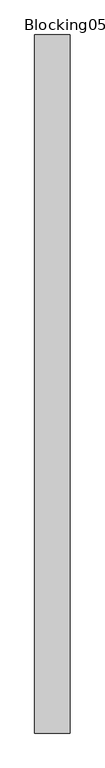
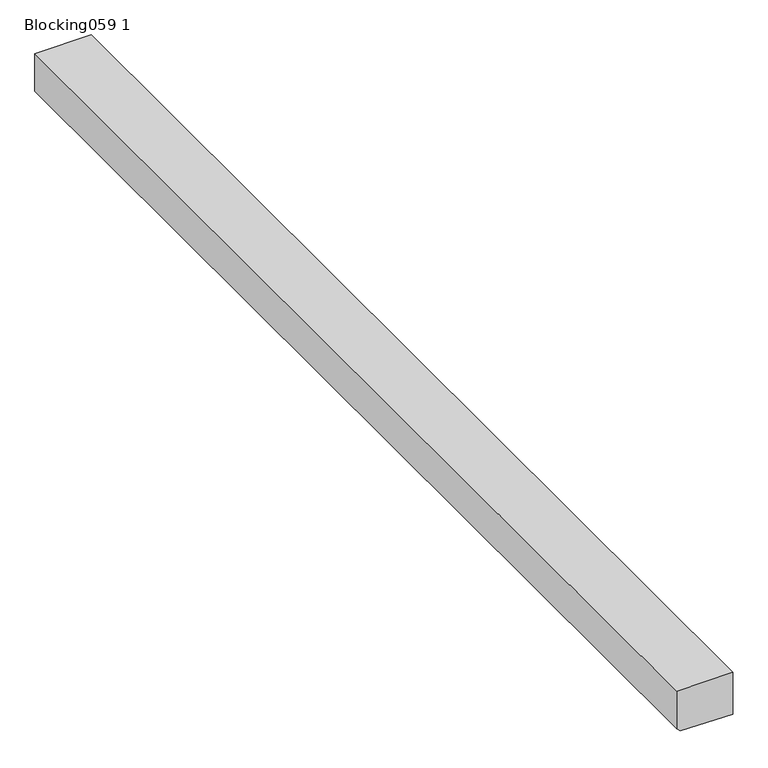
"""IFC4 building model written with IfcOpenShell, lengths in millimetres: proxy geometry, Blocking059 1 : Blocking059 1918."""

import ifcopenshell
import ifcopenshell.guid

model = None  # the IFC model being written
_history = None  # IfcOwnerHistory: only IFC2X3 demands one
_inside = {}  # id of a spatial element -> (the spatial element, [elements in it])
_under = {}  # id of a project, library or spatial element -> (it, [spatial elements below it])
_declared = {}  # id of a project -> (the project, [libraries it declares])
_typed = {}  # id of a type object -> (the type object, [elements of that type])
_made_of = {}  # id of a material, layer set ... -> (it, [elements and type objects made of it])


def new_model(schema):
    """Start an empty IFC model of exactly this schema.

    Asked for "IFC4X3", IfcOpenShell would pick the latest addendum, in which some entities
    have other attributes; the version numbers below select the first issue.
    IFC2X3 requires an IfcOwnerHistory on every rooted entity: one is made here for all.
    """
    global model, _history
    if schema == "IFC4X3":
        model = ifcopenshell.file(schema_version=(4, 3, 0, 0))
    else:
        model = ifcopenshell.file(schema=schema)
    _inside.clear()
    _under.clear()
    _declared.clear()
    _typed.clear()
    _made_of.clear()
    _history = None
    if model.schema == "IFC2X3":
        org = make("IfcOrganization", Name="unknown")
        user = make(
            "IfcPersonAndOrganization",
            ThePerson=make("IfcPerson", FamilyName="unknown"),
            TheOrganization=org,
        )
        app = make(
            "IfcApplication",
            ApplicationDeveloper=org,
            Version="unknown",
            ApplicationFullName="unknown",
            ApplicationIdentifier="unknown",
        )
        _history = make(
            "IfcOwnerHistory",
            OwningUser=user,
            OwningApplication=app,
            ChangeAction="ADDED",
            CreationDate=0,
        )
    return model


def make(cls, **values):
    """One entity of the class cls with the attributes given. An attribute that is None is left unset."""
    return model.create_entity(
        cls, **{name: value for name, value in values.items() if value is not None}
    )


def rooted(cls, **values):
    """An entity with a GlobalId (a new one), such as an element, a storey or a relation."""
    return make(cls, GlobalId=ifcopenshell.guid.new(), OwnerHistory=_history, **values)


def si_unit(unit_type, name, prefix=None):
    """IfcSIUnit, for example si_unit("LENGTHUNIT", "METRE", prefix="MILLI")."""
    return make("IfcSIUnit", UnitType=unit_type, Prefix=prefix, Name=name)


def assignment(units):
    """IfcUnitAssignment: the units of a project."""
    return None if units is None else make("IfcUnitAssignment", Units=units)


def point(xyz):
    """IfcCartesianPoint."""
    return None if xyz is None else make("IfcCartesianPoint", Coordinates=xyz)


def direction(xyz):
    """IfcDirection."""
    return None if xyz is None else make("IfcDirection", DirectionRatios=xyz)


def frame(location, z_axis=None, x_axis=None):
    """IfcAxis2Placement3D, a coordinate frame: its origin and axes. An axis left out is left unset."""
    return make(
        "IfcAxis2Placement3D",
        Location=point(location),
        Axis=direction(z_axis),
        RefDirection=direction(x_axis),
    )


def origin():
    """The frame at (0, 0, 0) with its axes left unset."""
    return frame((0.0, 0.0, 0.0))


def place(relative_to, where):
    """IfcLocalPlacement: puts the frame where relative to a parent placement (None: the world)."""
    return make(
        "IfcLocalPlacement", PlacementRelTo=relative_to, RelativePlacement=where
    )


def context(
    kind, dimensions, precision=None, world=None, true_north=None, identifier=None
):
    """IfcGeometricRepresentationContext, for example the 3D "Model" context."""
    return make(
        "IfcGeometricRepresentationContext",
        ContextIdentifier=identifier,
        ContextType=kind,
        CoordinateSpaceDimension=dimensions,
        Precision=precision,
        WorldCoordinateSystem=world,
        TrueNorth=true_north,
    )


def project(units=None, contexts=None):
    """IfcProject with its units and contexts."""
    return rooted(
        "IfcProject",
        Name="project",
        RepresentationContexts=contexts,
        UnitsInContext=assignment(units),
    )


def spatial(cls, under=None, at=None, **own):
    """A site, building, storey or space (cls), placed at a placement, below another one or the project."""
    s = rooted(cls, ObjectPlacement=at, **own)
    if under is not None:
        _under.setdefault(under.id(), (under, []))[1].append(s)
    return s


def polyline(points):
    """IfcPolyline through the points."""
    return make("IfcPolyline", Points=[point(p) for p in points])


def outline(outer, holes=None, kind="AREA"):
    """IfcArbitraryClosedProfileDef: a profile drawn as a closed curve; with holes, ...WithVoids."""
    if holes is None:
        return make("IfcArbitraryClosedProfileDef", ProfileType=kind, OuterCurve=outer)
    return make(
        "IfcArbitraryProfileDefWithVoids",
        ProfileType=kind,
        OuterCurve=outer,
        InnerCurves=holes,
    )


def extrude(swept, where, along, depth):
    """IfcExtrudedAreaSolid: the profile swept, set in the frame where, extruded along a direction by depth."""
    return make(
        "IfcExtrudedAreaSolid",
        SweptArea=swept,
        Position=where,
        ExtrudedDirection=direction(along),
        Depth=depth,
    )


def shape(context_of_items, identifier, shape_type, items):
    """IfcShapeRepresentation: the items that make up one representation, for example the "Body"."""
    return make(
        "IfcShapeRepresentation",
        ContextOfItems=context_of_items,
        RepresentationIdentifier=identifier,
        RepresentationType=shape_type,
        Items=items,
    )


def source(mapping_origin, context_of_items, identifier, shape_type, items):
    """IfcRepresentationMap: a shape defined once, which mapped items show again and again."""
    return make(
        "IfcRepresentationMap",
        MappingOrigin=mapping_origin,
        MappedRepresentation=shape(context_of_items, identifier, shape_type, items),
    )


def transform(
    local_origin,
    x_axis=None,
    y_axis=None,
    z_axis=None,
    scale=None,
    scale2=None,
    scale3=None,
    uniform=True,
):
    """IfcCartesianTransformationOperator3D, or its non-uniform kind. x_axis, y_axis, z_axis: its Axis1, 2, 3."""
    if uniform:
        return make(
            "IfcCartesianTransformationOperator3D",
            Axis1=direction(x_axis),
            Axis2=direction(y_axis),
            LocalOrigin=point(local_origin),
            Scale=scale,
            Axis3=direction(z_axis),
        )
    return make(
        "IfcCartesianTransformationOperator3DnonUniform",
        Axis1=direction(x_axis),
        Axis2=direction(y_axis),
        LocalOrigin=point(local_origin),
        Scale=scale,
        Axis3=direction(z_axis),
        Scale2=scale2,
        Scale3=scale3,
    )


def mapped(mapping_source, mapping_target):
    """IfcMappedItem: shows the shape of a source again, moved by a transform."""
    return make(
        "IfcMappedItem", MappingSource=mapping_source, MappingTarget=mapping_target
    )


def made_of(thing, what):
    """Note that an element or type object is made of a material, layer set ...; save() writes the relation."""
    if what is not None:
        _made_of.setdefault(what.id(), (what, []))[1].append(thing)
    return thing


def element(
    cls,
    number,
    at=None,
    inside=None,
    cuts=None,
    type_object=None,
    material=None,
    context=None,
    identifier="Body",
    shape_type=None,
    held_by="IfcProductDefinitionShape",
    body=None,
    shapes=None,
    **own,
):
    """One element of the class cls, such as IfcWall. Its Tag is "e" and its number.

    at: its placement. inside: the storey or other place that contains it. cuts: it is an
    opening in that element (IfcRelVoidsElement). A single representation is given by context,
    identifier, shape_type and body (its items); several are given by shapes. held_by: the class
    of the entity that holds the representations. save() writes the other relations.
    """
    e = rooted(cls, Tag="e%d" % number, ObjectPlacement=at, **own)
    if body is not None:
        shapes = [shape(context, identifier, shape_type, body)]
    if shapes is not None:
        e.Representation = make(held_by, Representations=shapes)
    if inside is not None:
        _inside.setdefault(inside.id(), (inside, []))[1].append(e)
    if cuts is not None:
        rooted(
            "IfcRelVoidsElement", RelatingBuildingElement=cuts, RelatedOpeningElement=e
        )
    if type_object is not None:
        _typed.setdefault(type_object.id(), (type_object, []))[1].append(e)
    return made_of(e, material)


def aggregate(whole, parts):
    """IfcRelAggregates: a whole, such as a stair, and the parts it consists of."""
    return rooted("IfcRelAggregates", RelatingObject=whole, RelatedObjects=parts)


def save(model, path):
    """Write the relations noted so far, then the file.

    IfcRelAggregates (storeys below a building ...), IfcRelContainedInSpatialStructure (elements
    in a storey), IfcRelDefinesByType, IfcRelAssociatesMaterial and IfcRelDeclares: one each for
    every whole, place, type object, material and project.
    """
    for whole, parts in _under.values():
        aggregate(whole, parts)
    for where, things in _inside.values():
        rooted(
            "IfcRelContainedInSpatialStructure",
            RelatedElements=things,
            RelatingStructure=where,
        )
    for kind, things in _typed.values():
        rooted("IfcRelDefinesByType", RelatedObjects=things, RelatingType=kind)
    for what, things in _made_of.values():
        rooted("IfcRelAssociatesMaterial", RelatedObjects=things, RelatingMaterial=what)
    for by, libraries in _declared.values():
        rooted("IfcRelDeclares", RelatingContext=by, RelatedDefinitions=libraries)
    model.write(path)


def blocking059_1_d2a3d8a8(model_context):
    return source(origin(), model_context, "Body", "SweptSolid", [
        extrude(outline(polyline([(40118.3092895, -7012.6070533), (40118.3092895, -7114.2070533), (40047.0174737, -7114.2070533), (40040.2769302, -7107.5750792), (40038.291814, -7012.6070533), (40118.3092895, -7012.6070533)])), frame((0.0, 7182.1531721, 0.0), z_axis=(0.0, 1.0, 0.0), x_axis=(0.0, 0.0, 1.0)), (0.0, 0.0, 1.0), 2000.0),
    ])


if __name__ == "__main__":
    model = new_model("IFC4")
    model_context = context("Model", 3, world=origin())
    ifc_project = project(units=[si_unit("LENGTHUNIT", "METRE", prefix="MILLI")], contexts=[model_context])
    site = spatial("IfcSite", under=ifc_project)
    building = spatial("IfcBuilding", under=site)
    placement = place(None, origin())
    blocking059_1_shape = blocking059_1_d2a3d8a8(model_context)
    element("IfcBuildingElementProxy", 1, Name="Blocking059 1 : Blocking059 1918", ObjectType="Blocking059 1 : Blocking059 1918", at=placement, inside=building, context=model_context, shape_type="MappedRepresentation", body=[
        mapped(blocking059_1_shape, transform((0.0, 0.0, 0.0), x_axis=(1.0, 0.0, 0.0), y_axis=(0.0, 1.0, 0.0), z_axis=(0.0, 0.0, 1.0))),
    ])
    save(model, "model.ifc")

# Revit data of these elements
# Type "Blocking059 1 : Blocking059 1918"
#   NameOverride = "Blocking059"
# Element 1 (IfcBuildingElementProxy, "Blocking059 1 : Blocking059 1918")
#   Materials on its faces: "TREATED INTERMITTENT (FOR DRAINAGE) BLOCKING - SET IN BED OF SEALANT"
# Materials
#   "TREATED INTERMITTENT (FOR DRAINAGE) BLOCKING - SET IN BED OF SEALANT": class "Unassigned", colour RGB 140 161 107, transparency 0, Cost = 0
